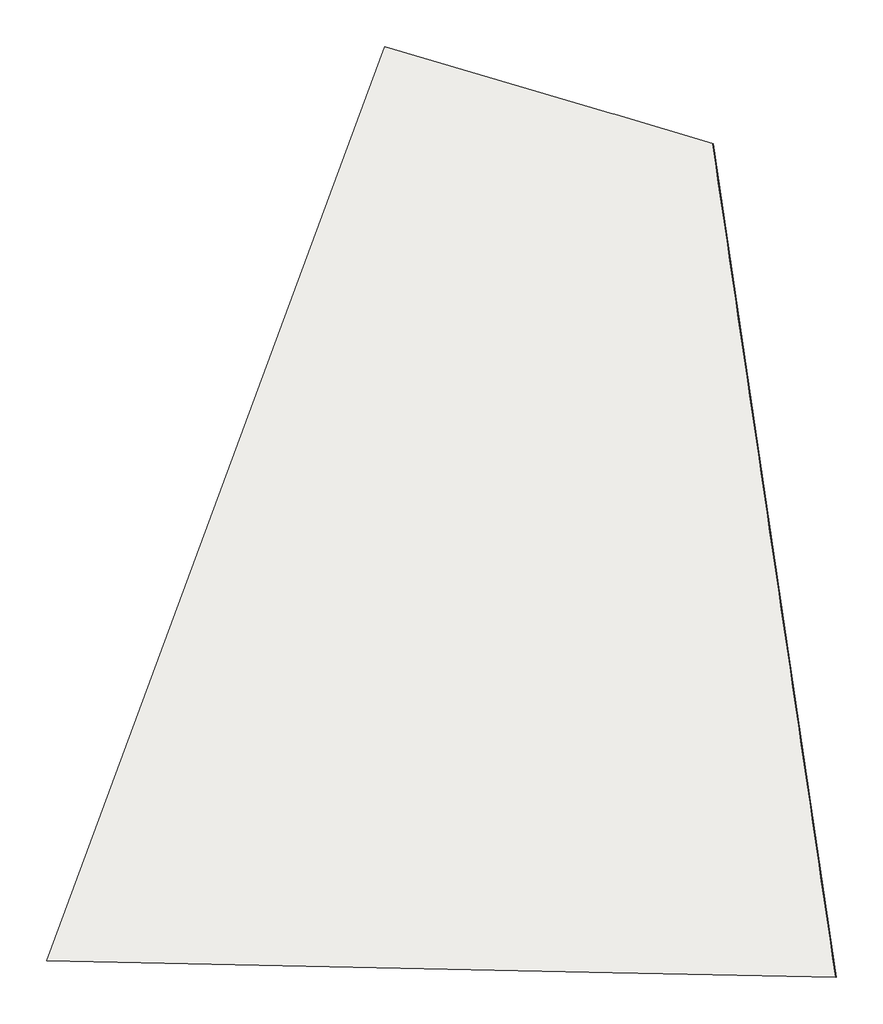
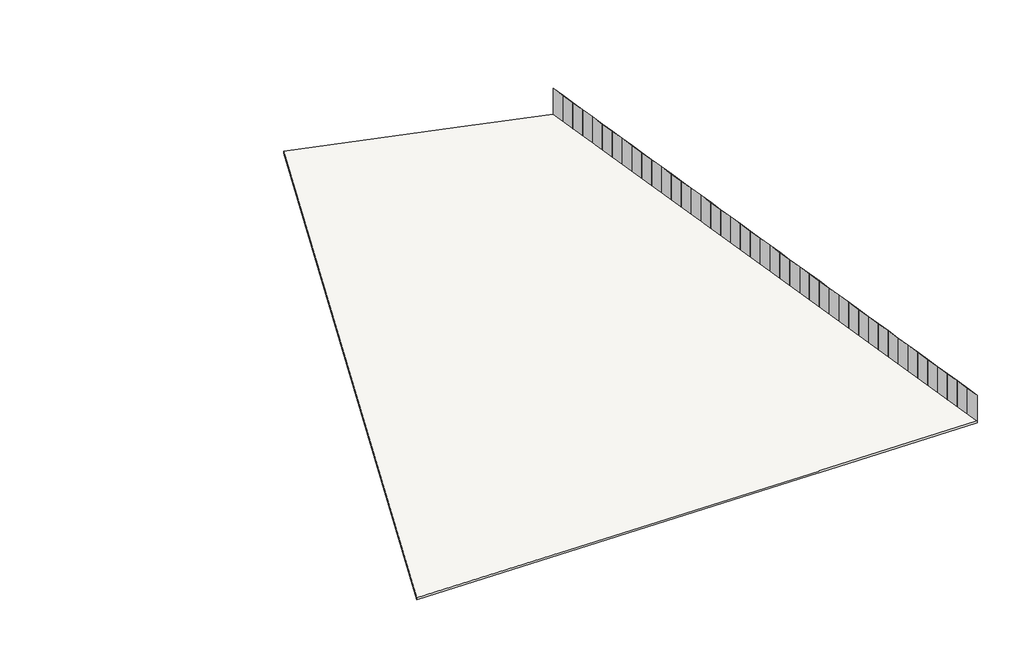
# One storey: 44 plates, 1 slab.
"""IFC4 building model written with IfcOpenShell, lengths in millimetres."""

import ifcopenshell
import ifcopenshell.guid

model = None  # the IFC model being written
_history = None  # IfcOwnerHistory: only IFC2X3 demands one
_inside = {}  # id of a spatial element -> (the spatial element, [elements in it])
_under = {}  # id of a project, library or spatial element -> (it, [spatial elements below it])
_declared = {}  # id of a project -> (the project, [libraries it declares])
_typed = {}  # id of a type object -> (the type object, [elements of that type])
_made_of = {}  # id of a material, layer set ... -> (it, [elements and type objects made of it])


def new_model(schema):
    """Start an empty IFC model of exactly this schema.

    Asked for "IFC4X3", IfcOpenShell would pick the latest addendum, in which some entities
    have other attributes; the version numbers below select the first issue.
    IFC2X3 requires an IfcOwnerHistory on every rooted entity: one is made here for all.
    """
    global model, _history
    if schema == "IFC4X3":
        model = ifcopenshell.file(schema_version=(4, 3, 0, 0))
    else:
        model = ifcopenshell.file(schema=schema)
    _inside.clear()
    _under.clear()
    _declared.clear()
    _typed.clear()
    _made_of.clear()
    _history = None
    if model.schema == "IFC2X3":
        org = make("IfcOrganization", Name="unknown")
        user = make(
            "IfcPersonAndOrganization",
            ThePerson=make("IfcPerson", FamilyName="unknown"),
            TheOrganization=org,
        )
        app = make(
            "IfcApplication",
            ApplicationDeveloper=org,
            Version="unknown",
            ApplicationFullName="unknown",
            ApplicationIdentifier="unknown",
        )
        _history = make(
            "IfcOwnerHistory",
            OwningUser=user,
            OwningApplication=app,
            ChangeAction="ADDED",
            CreationDate=0,
        )
    return model


def make(cls, **values):
    """One entity of the class cls with the attributes given. An attribute that is None is left unset."""
    return model.create_entity(
        cls, **{name: value for name, value in values.items() if value is not None}
    )


def rooted(cls, **values):
    """An entity with a GlobalId (a new one), such as an element, a storey or a relation."""
    return make(cls, GlobalId=ifcopenshell.guid.new(), OwnerHistory=_history, **values)


def si_unit(unit_type, name, prefix=None):
    """IfcSIUnit, for example si_unit("LENGTHUNIT", "METRE", prefix="MILLI")."""
    return make("IfcSIUnit", UnitType=unit_type, Prefix=prefix, Name=name)


def assignment(units):
    """IfcUnitAssignment: the units of a project."""
    return None if units is None else make("IfcUnitAssignment", Units=units)


def point(xyz):
    """IfcCartesianPoint."""
    return None if xyz is None else make("IfcCartesianPoint", Coordinates=xyz)


def direction(xyz):
    """IfcDirection."""
    return None if xyz is None else make("IfcDirection", DirectionRatios=xyz)


def frame(location, z_axis=None, x_axis=None):
    """IfcAxis2Placement3D, a coordinate frame: its origin and axes. An axis left out is left unset."""
    return make(
        "IfcAxis2Placement3D",
        Location=point(location),
        Axis=direction(z_axis),
        RefDirection=direction(x_axis),
    )


def origin():
    """The frame at (0, 0, 0) with its axes left unset."""
    return frame((0.0, 0.0, 0.0))


def origin_with_axes():
    """The frame at (0, 0, 0) with the z axis (0, 0, 1) and the x axis (1, 0, 0) written out."""
    return frame((0.0, 0.0, 0.0), z_axis=(0.0, 0.0, 1.0), x_axis=(1.0, 0.0, 0.0))


def place(relative_to, where):
    """IfcLocalPlacement: puts the frame where relative to a parent placement (None: the world)."""
    return make(
        "IfcLocalPlacement", PlacementRelTo=relative_to, RelativePlacement=where
    )


def context(
    kind, dimensions, precision=None, world=None, true_north=None, identifier=None
):
    """IfcGeometricRepresentationContext, for example the 3D "Model" context."""
    return make(
        "IfcGeometricRepresentationContext",
        ContextIdentifier=identifier,
        ContextType=kind,
        CoordinateSpaceDimension=dimensions,
        Precision=precision,
        WorldCoordinateSystem=world,
        TrueNorth=true_north,
    )


def project(units=None, contexts=None):
    """IfcProject with its units and contexts."""
    return rooted(
        "IfcProject",
        Name="project",
        RepresentationContexts=contexts,
        UnitsInContext=assignment(units),
    )


def spatial(cls, under=None, at=None, **own):
    """A site, building, storey or space (cls), placed at a placement, below another one or the project."""
    s = rooted(cls, ObjectPlacement=at, **own)
    if under is not None:
        _under.setdefault(under.id(), (under, []))[1].append(s)
    return s


def polyline(points):
    """IfcPolyline through the points."""
    return make("IfcPolyline", Points=[point(p) for p in points])


def outline(outer, holes=None, kind="AREA"):
    """IfcArbitraryClosedProfileDef: a profile drawn as a closed curve; with holes, ...WithVoids."""
    if holes is None:
        return make("IfcArbitraryClosedProfileDef", ProfileType=kind, OuterCurve=outer)
    return make(
        "IfcArbitraryProfileDefWithVoids",
        ProfileType=kind,
        OuterCurve=outer,
        InnerCurves=holes,
    )


def extrude(swept, where, along, depth):
    """IfcExtrudedAreaSolid: the profile swept, set in the frame where, extruded along a direction by depth."""
    return make(
        "IfcExtrudedAreaSolid",
        SweptArea=swept,
        Position=where,
        ExtrudedDirection=direction(along),
        Depth=depth,
    )


def faces_of(points, faces, orient=None, outer=None):
    """IfcFace entities. A face is a list of loops; a loop is a list of indices into points, from 0.

    orient and outer hold one flag for each loop. By default every Orientation is true, the
    first loop of a face is its IfcFaceOuterBound and the others are IfcFaceBound.
    """
    made = []
    for i, loops in enumerate(faces):
        bounds = []
        for j, loop in enumerate(loops):
            is_outer = j == 0 if outer is None else outer[i][j]
            bounds.append(
                make(
                    "IfcFaceOuterBound" if is_outer else "IfcFaceBound",
                    Bound=make("IfcPolyLoop", Polygon=[points[k] for k in loop]),
                    Orientation=True if orient is None else orient[i][j],
                )
            )
        made.append(make("IfcFace", Bounds=bounds))
    return made


def faceted_brep(points, faces, orient=None, outer=None, voids=None):
    """IfcFacetedBrep: a solid bounded by flat faces; with voids (closed shells), ...WithVoids."""
    shared = [point(p) for p in points]
    hull = make("IfcClosedShell", CfsFaces=faces_of(shared, faces, orient, outer))
    if voids is None:
        return make("IfcFacetedBrep", Outer=hull)
    return make(
        "IfcFacetedBrepWithVoids",
        Outer=hull,
        Voids=[
            make(cls, CfsFaces=faces_of(shared, fs, o, b)) for cls, fs, o, b in voids
        ],
    )


def shape(context_of_items, identifier, shape_type, items):
    """IfcShapeRepresentation: the items that make up one representation, for example the "Body"."""
    return make(
        "IfcShapeRepresentation",
        ContextOfItems=context_of_items,
        RepresentationIdentifier=identifier,
        RepresentationType=shape_type,
        Items=items,
    )


def source(mapping_origin, context_of_items, identifier, shape_type, items):
    """IfcRepresentationMap: a shape defined once, which mapped items show again and again."""
    return make(
        "IfcRepresentationMap",
        MappingOrigin=mapping_origin,
        MappedRepresentation=shape(context_of_items, identifier, shape_type, items),
    )


def transform(
    local_origin,
    x_axis=None,
    y_axis=None,
    z_axis=None,
    scale=None,
    scale2=None,
    scale3=None,
    uniform=True,
):
    """IfcCartesianTransformationOperator3D, or its non-uniform kind. x_axis, y_axis, z_axis: its Axis1, 2, 3."""
    if uniform:
        return make(
            "IfcCartesianTransformationOperator3D",
            Axis1=direction(x_axis),
            Axis2=direction(y_axis),
            LocalOrigin=point(local_origin),
            Scale=scale,
            Axis3=direction(z_axis),
        )
    return make(
        "IfcCartesianTransformationOperator3DnonUniform",
        Axis1=direction(x_axis),
        Axis2=direction(y_axis),
        LocalOrigin=point(local_origin),
        Scale=scale,
        Axis3=direction(z_axis),
        Scale2=scale2,
        Scale3=scale3,
    )


def mapped(mapping_source, mapping_target):
    """IfcMappedItem: shows the shape of a source again, moved by a transform."""
    return make(
        "IfcMappedItem", MappingSource=mapping_source, MappingTarget=mapping_target
    )


def made_of(thing, what):
    """Note that an element or type object is made of a material, layer set ...; save() writes the relation."""
    if what is not None:
        _made_of.setdefault(what.id(), (what, []))[1].append(thing)
    return thing


def element(
    cls,
    number,
    at=None,
    inside=None,
    cuts=None,
    type_object=None,
    material=None,
    context=None,
    identifier="Body",
    shape_type=None,
    held_by="IfcProductDefinitionShape",
    body=None,
    shapes=None,
    **own,
):
    """One element of the class cls, such as IfcWall. Its Tag is "e" and its number.

    at: its placement. inside: the storey or other place that contains it. cuts: it is an
    opening in that element (IfcRelVoidsElement). A single representation is given by context,
    identifier, shape_type and body (its items); several are given by shapes. held_by: the class
    of the entity that holds the representations. save() writes the other relations.
    """
    e = rooted(cls, Tag="e%d" % number, ObjectPlacement=at, **own)
    if body is not None:
        shapes = [shape(context, identifier, shape_type, body)]
    if shapes is not None:
        e.Representation = make(held_by, Representations=shapes)
    if inside is not None:
        _inside.setdefault(inside.id(), (inside, []))[1].append(e)
    if cuts is not None:
        rooted(
            "IfcRelVoidsElement", RelatingBuildingElement=cuts, RelatedOpeningElement=e
        )
    if type_object is not None:
        _typed.setdefault(type_object.id(), (type_object, []))[1].append(e)
    return made_of(e, material)


def aggregate(whole, parts):
    """IfcRelAggregates: a whole, such as a stair, and the parts it consists of."""
    return rooted("IfcRelAggregates", RelatingObject=whole, RelatedObjects=parts)


def save(model, path):
    """Write the relations noted so far, then the file.

    IfcRelAggregates (storeys below a building ...), IfcRelContainedInSpatialStructure (elements
    in a storey), IfcRelDefinesByType, IfcRelAssociatesMaterial and IfcRelDeclares: one each for
    every whole, place, type object, material and project.
    """
    for whole, parts in _under.values():
        aggregate(whole, parts)
    for where, things in _inside.values():
        rooted(
            "IfcRelContainedInSpatialStructure",
            RelatedElements=things,
            RelatingStructure=where,
        )
    for kind, things in _typed.values():
        rooted("IfcRelDefinesByType", RelatedObjects=things, RelatingType=kind)
    for what, things in _made_of.values():
        rooted("IfcRelAssociatesMaterial", RelatedObjects=things, RelatingMaterial=what)
    for by, libraries in _declared.values():
        rooted("IfcRelDeclares", RelatingContext=by, RelatedDefinitions=libraries)
    model.write(path)


def painel_do_sistema_1cdad03e(model_context):
    return source(origin(), model_context, "Body", "SweptSolid", [
        extrude(outline(polyline([(1500.0, 24.5), (-1500.0, 24.5), (-1500.0, 49.5), (1500.0, 49.5), (1500.0, 24.5)])), origin_with_axes(), (0.0, 0.0, 1.0), 1500.0),
    ])


def painel_do_sistema_1cb3a730(model_context):
    return source(origin(), model_context, "Body", "SweptSolid", [
        extrude(outline(polyline([(1500.0, 24.5), (-1500.0, 24.5), (-1500.0, 49.5), (1500.0, 49.5), (1500.0, 24.5)])), origin_with_axes(), (0.0, 0.0, 1.0), 20.0931032),
    ])


model = new_model("IFC4")

# Units and contexts
model_context = context("Model", 3, world=origin())
ifc_project = project(units=[si_unit("LENGTHUNIT", "METRE", prefix="MILLI")], contexts=[model_context])

# Site, building, storey
site = spatial("IfcSite", under=ifc_project)
building = spatial("IfcBuilding", under=site)
storey = spatial("IfcBuildingStorey", under=building, Name="Nível 7", Elevation=6000.0)

# Plates
placement = place(None, origin())
painel_do_sistema_shape = painel_do_sistema_1cdad03e(model_context)
element("IfcPlate", 1, ObjectType="Painel do sistema : Envidraçado", at=placement, inside=storey, context=model_context, shape_type="MappedRepresentation", body=[
    mapped(painel_do_sistema_shape, transform((27835.0106579, -36774.1442579, 7500.000015), x_axis=(0.0, 0.0, 1.0), y_axis=(-0.9892699032546327, -0.1460994815684493, 0.0), z_axis=(0.1460994815684493, -0.9892699032546327, 0.0))),
])
element("IfcPlate", 2, ObjectType="Painel do sistema : Envidraçado", at=placement, inside=storey, context=model_context, shape_type="MappedRepresentation", body=[
    mapped(painel_do_sistema_shape, transform((27615.8614356, -35290.239403, 7500.000015), x_axis=(0.0, 0.0, 1.0), y_axis=(-0.9892699032546328, -0.14609948156844885, 0.0), z_axis=(0.14609948156844885, -0.9892699032546328, 0.0))),
])
element("IfcPlate", 3, ObjectType="Painel do sistema : Envidraçado", at=placement, inside=storey, context=model_context, shape_type="MappedRepresentation", body=[
    mapped(painel_do_sistema_shape, transform((27396.7122132, -33806.3345481, 7500.000015), x_axis=(0.0, 0.0, 1.0), y_axis=(-0.9892699032546323, -0.1460994815684521, 0.0), z_axis=(0.1460994815684521, -0.9892699032546323, 0.0))),
])
element("IfcPlate", 4, ObjectType="Painel do sistema : Envidraçado", at=placement, inside=storey, context=model_context, shape_type="MappedRepresentation", body=[
    mapped(painel_do_sistema_shape, transform((27177.5629909, -32322.4296932, 7500.000015), x_axis=(0.0, 0.0, 1.0), y_axis=(-0.9892699032546328, -0.14609948156844926, 0.0), z_axis=(0.14609948156844926, -0.9892699032546328, 0.0))),
])
element("IfcPlate", 5, ObjectType="Painel do sistema : Envidraçado", at=placement, inside=storey, context=model_context, shape_type="MappedRepresentation", body=[
    mapped(painel_do_sistema_shape, transform((26958.4137685, -30838.5248383, 7500.000015), x_axis=(0.0, 0.0, 1.0), y_axis=(-0.9892699032546327, -0.1460994815684493, 0.0), z_axis=(0.1460994815684493, -0.9892699032546327, 0.0))),
])
element("IfcPlate", 6, ObjectType="Painel do sistema : Envidraçado", at=placement, inside=storey, context=model_context, shape_type="MappedRepresentation", body=[
    mapped(painel_do_sistema_shape, transform((26739.2645462, -29354.6199835, 7500.000015), x_axis=(0.0, 0.0, 1.0), y_axis=(-0.9892699032546327, -0.1460994815684493, 0.0), z_axis=(0.1460994815684493, -0.9892699032546327, 0.0))),
])
element("IfcPlate", 7, ObjectType="Painel do sistema : Envidraçado", at=placement, inside=storey, context=model_context, shape_type="MappedRepresentation", body=[
    mapped(painel_do_sistema_shape, transform((26520.1153238, -27870.7151286, 7500.000015), x_axis=(0.0, 0.0, 1.0), y_axis=(-0.9892699032546324, -0.1460994815684517, 0.0), z_axis=(0.1460994815684517, -0.9892699032546324, 0.0))),
])
element("IfcPlate", 8, ObjectType="Painel do sistema : Envidraçado", at=placement, inside=storey, context=model_context, shape_type="MappedRepresentation", body=[
    mapped(painel_do_sistema_shape, transform((26300.9661014, -26386.8102737, 7500.000015), x_axis=(0.0, 0.0, 1.0), y_axis=(-0.9892699032546327, -0.1460994815684493, 0.0), z_axis=(0.1460994815684493, -0.9892699032546327, 0.0))),
])
element("IfcPlate", 9, ObjectType="Painel do sistema : Envidraçado", at=placement, inside=storey, context=model_context, shape_type="MappedRepresentation", body=[
    mapped(painel_do_sistema_shape, transform((26081.8168791, -24902.9054188, 7500.000015), x_axis=(0.0, 0.0, 1.0), y_axis=(-0.9892699032546328, -0.14609948156844887, 0.0), z_axis=(0.14609948156844887, -0.9892699032546328, 0.0))),
])
element("IfcPlate", 10, ObjectType="Painel do sistema : Envidraçado", at=placement, inside=storey, context=model_context, shape_type="MappedRepresentation", body=[
    mapped(painel_do_sistema_shape, transform((25862.6676567, -23419.0005639, 7500.000015), x_axis=(0.0, 0.0, 1.0), y_axis=(-0.9892699032546324, -0.1460994815684517, 0.0), z_axis=(0.1460994815684517, -0.9892699032546324, 0.0))),
])
element("IfcPlate", 11, ObjectType="Painel do sistema : Envidraçado", at=placement, inside=storey, context=model_context, shape_type="MappedRepresentation", body=[
    mapped(painel_do_sistema_shape, transform((25643.5184344, -21935.095709, 7500.000015), x_axis=(0.0, 0.0, 1.0), y_axis=(-0.9892699032546327, -0.14609948156844926, 0.0), z_axis=(0.14609948156844926, -0.9892699032546327, 0.0))),
])
element("IfcPlate", 12, ObjectType="Painel do sistema : Envidraçado", at=placement, inside=storey, context=model_context, shape_type="MappedRepresentation", body=[
    mapped(painel_do_sistema_shape, transform((25424.369212, -20451.1908542, 7500.000015), x_axis=(0.0, 0.0, 1.0), y_axis=(-0.9892699032546324, -0.1460994815684517, 0.0), z_axis=(0.1460994815684517, -0.9892699032546324, 0.0))),
])
element("IfcPlate", 13, ObjectType="Painel do sistema : Envidraçado", at=placement, inside=storey, context=model_context, shape_type="MappedRepresentation", body=[
    mapped(painel_do_sistema_shape, transform((25205.2199897, -18967.2859993, 7500.000015), x_axis=(0.0, 0.0, 1.0), y_axis=(-0.9892699032546328, -0.14609948156844865, 0.0), z_axis=(0.14609948156844865, -0.9892699032546328, 0.0))),
])
element("IfcPlate", 14, ObjectType="Painel do sistema : Envidraçado", at=placement, inside=storey, context=model_context, shape_type="MappedRepresentation", body=[
    mapped(painel_do_sistema_shape, transform((24986.0707673, -17483.3811444, 7500.000015), x_axis=(0.0, 0.0, 1.0), y_axis=(-0.9892699032546328, -0.1460994815684491, 0.0), z_axis=(0.1460994815684491, -0.9892699032546328, 0.0))),
])
element("IfcPlate", 15, ObjectType="Painel do sistema : Envidraçado", at=placement, inside=storey, context=model_context, shape_type="MappedRepresentation", body=[
    mapped(painel_do_sistema_shape, transform((24766.921545, -15999.4762895, 7500.000015), x_axis=(0.0, 0.0, 1.0), y_axis=(-0.9892699032546327, -0.1460994815684493, 0.0), z_axis=(0.1460994815684493, -0.9892699032546327, 0.0))),
])
element("IfcPlate", 16, ObjectType="Painel do sistema : Envidraçado", at=placement, inside=storey, context=model_context, shape_type="MappedRepresentation", body=[
    mapped(painel_do_sistema_shape, transform((24547.7723226, -14515.5714346, 7500.000015), x_axis=(0.0, 0.0, 1.0), y_axis=(-0.9892699032546324, -0.1460994815684517, 0.0), z_axis=(0.1460994815684517, -0.9892699032546324, 0.0))),
])
element("IfcPlate", 17, ObjectType="Painel do sistema : Envidraçado", at=placement, inside=storey, context=model_context, shape_type="MappedRepresentation", body=[
    mapped(painel_do_sistema_shape, transform((24328.6231003, -13031.6665798, 7500.000015), x_axis=(0.0, 0.0, 1.0), y_axis=(-0.9892699032546327, -0.1460994815684495, 0.0), z_axis=(0.1460994815684495, -0.9892699032546327, 0.0))),
])
element("IfcPlate", 18, ObjectType="Painel do sistema : Envidraçado", at=placement, inside=storey, context=model_context, shape_type="MappedRepresentation", body=[
    mapped(painel_do_sistema_shape, transform((24109.4738779, -11547.7617249, 7500.000015), x_axis=(0.0, 0.0, 1.0), y_axis=(-0.9892699032546328, -0.1460994815684491, 0.0), z_axis=(0.1460994815684491, -0.9892699032546328, 0.0))),
])
element("IfcPlate", 19, ObjectType="Painel do sistema : Envidraçado", at=placement, inside=storey, context=model_context, shape_type="MappedRepresentation", body=[
    mapped(painel_do_sistema_shape, transform((23890.3246556, -10063.85687, 7500.000015), x_axis=(0.0, 0.0, 1.0), y_axis=(-0.9892699032546324, -0.14609948156845148, 0.0), z_axis=(0.14609948156845148, -0.9892699032546324, 0.0))),
])
element("IfcPlate", 20, ObjectType="Painel do sistema : Envidraçado", at=placement, inside=storey, context=model_context, shape_type="MappedRepresentation", body=[
    mapped(painel_do_sistema_shape, transform((23671.1754332, -8579.9520151, 7500.000015), x_axis=(0.0, 0.0, 1.0), y_axis=(-0.9892699032546332, -0.14609948156844624, 0.0), z_axis=(0.14609948156844624, -0.9892699032546332, 0.0))),
])
element("IfcPlate", 21, ObjectType="Painel do sistema : Envidraçado", at=placement, inside=storey, context=model_context, shape_type="MappedRepresentation", body=[
    mapped(painel_do_sistema_shape, transform((23452.0262109, -7096.0471602, 7500.000015), x_axis=(0.0, 0.0, 1.0), y_axis=(-0.9892699032546319, -0.14609948156845473, 0.0), z_axis=(0.14609948156845473, -0.9892699032546319, 0.0))),
])
element("IfcPlate", 22, ObjectType="Painel do sistema : Envidraçado", at=placement, inside=storey, context=model_context, shape_type="MappedRepresentation", body=[
    mapped(painel_do_sistema_shape, transform((23232.8769885, -5612.1423053, 7500.000015), x_axis=(0.0, 0.0, 1.0), y_axis=(-0.9892699032546332, -0.1460994815684465, 0.0), z_axis=(0.1460994815684465, -0.9892699032546332, 0.0))),
])
element("IfcPlate", 23, ObjectType="Painel do sistema : Envidraçado", at=placement, inside=storey, context=model_context, shape_type="MappedRepresentation", body=[
    mapped(painel_do_sistema_shape, transform((23013.7277662, -4128.2374505, 7500.000015), x_axis=(0.0, 0.0, 1.0), y_axis=(-0.9892699032546324, -0.1460994815684517, 0.0), z_axis=(0.1460994815684517, -0.9892699032546324, 0.0))),
])
element("IfcPlate", 24, ObjectType="Painel do sistema : Envidraçado", at=placement, inside=storey, context=model_context, shape_type="MappedRepresentation", body=[
    mapped(painel_do_sistema_shape, transform((22794.5785438, -2644.3325956, 7500.000015), x_axis=(0.0, 0.0, 1.0), y_axis=(-0.9892699032546328, -0.14609948156844865, 0.0), z_axis=(0.14609948156844865, -0.9892699032546328, 0.0))),
])
element("IfcPlate", 25, ObjectType="Painel do sistema : Envidraçado", at=placement, inside=storey, context=model_context, shape_type="MappedRepresentation", body=[
    mapped(painel_do_sistema_shape, transform((22575.4293215, -1160.4277407, 7500.000015), x_axis=(0.0, 0.0, 1.0), y_axis=(-0.9892699032546327, -0.1460994815684493, 0.0), z_axis=(0.1460994815684493, -0.9892699032546327, 0.0))),
])
element("IfcPlate", 26, ObjectType="Painel do sistema : Envidraçado", at=placement, inside=storey, context=model_context, shape_type="MappedRepresentation", body=[
    mapped(painel_do_sistema_shape, transform((22356.2800991, 323.4771142, 7500.000015), x_axis=(0.0, 0.0, 1.0), y_axis=(-0.9892699032546324, -0.14609948156845148, 0.0), z_axis=(0.14609948156845148, -0.9892699032546324, 0.0))),
])
element("IfcPlate", 27, ObjectType="Painel do sistema : Envidraçado", at=placement, inside=storey, context=model_context, shape_type="MappedRepresentation", body=[
    mapped(painel_do_sistema_shape, transform((22137.1308767, 1807.3819691, 7500.000015), x_axis=(0.0, 0.0, 1.0), y_axis=(-0.9892699032546332, -0.1460994815684469, 0.0), z_axis=(0.1460994815684469, -0.9892699032546332, 0.0))),
])
element("IfcPlate", 28, ObjectType="Painel do sistema : Envidraçado", at=placement, inside=storey, context=model_context, shape_type="MappedRepresentation", body=[
    mapped(painel_do_sistema_shape, transform((21917.9816544, 3291.2868239, 7500.000015), x_axis=(0.0, 0.0, 1.0), y_axis=(-0.9892699032546323, -0.1460994815684521, 0.0), z_axis=(0.1460994815684521, -0.9892699032546323, 0.0))),
])
element("IfcPlate", 29, ObjectType="Painel do sistema : Envidraçado", at=placement, inside=storey, context=model_context, shape_type="MappedRepresentation", body=[
    mapped(painel_do_sistema_shape, transform((21698.832432, 4775.1916788, 7500.000015), x_axis=(0.0, 0.0, 1.0), y_axis=(-0.9892699032546323, -0.14609948156845234, 0.0), z_axis=(0.14609948156845234, -0.9892699032546323, 0.0))),
])
element("IfcPlate", 30, ObjectType="Painel do sistema : Envidraçado", at=placement, inside=storey, context=model_context, shape_type="MappedRepresentation", body=[
    mapped(painel_do_sistema_shape, transform((21479.6832097, 6259.0965337, 7500.000015), x_axis=(0.0, 0.0, 1.0), y_axis=(-0.9892699032546332, -0.1460994815684465, 0.0), z_axis=(0.1460994815684465, -0.9892699032546332, 0.0))),
])
element("IfcPlate", 31, ObjectType="Painel do sistema : Envidraçado", at=placement, inside=storey, context=model_context, shape_type="MappedRepresentation", body=[
    mapped(painel_do_sistema_shape, transform((21260.5339873, 7743.0013886, 7500.000015), x_axis=(0.0, 0.0, 1.0), y_axis=(-0.9892699032546323, -0.14609948156845234, 0.0), z_axis=(0.14609948156845234, -0.9892699032546323, 0.0))),
])
element("IfcPlate", 32, ObjectType="Painel do sistema : Envidraçado", at=placement, inside=storey, context=model_context, shape_type="MappedRepresentation", body=[
    mapped(painel_do_sistema_shape, transform((21041.384765, 9226.9062435, 7500.000015), x_axis=(0.0, 0.0, 1.0), y_axis=(-0.9892699032546327, -0.1460994815684495, 0.0), z_axis=(0.1460994815684495, -0.9892699032546327, 0.0))),
])
element("IfcPlate", 33, ObjectType="Painel do sistema : Envidraçado", at=placement, inside=storey, context=model_context, shape_type="MappedRepresentation", body=[
    mapped(painel_do_sistema_shape, transform((20822.2355426, 10710.8110984, 7500.000015), x_axis=(0.0, 0.0, 1.0), y_axis=(-0.9892699032546327, -0.1460994815684495, 0.0), z_axis=(0.1460994815684495, -0.9892699032546327, 0.0))),
])
element("IfcPlate", 34, ObjectType="Painel do sistema : Envidraçado", at=placement, inside=storey, context=model_context, shape_type="MappedRepresentation", body=[
    mapped(painel_do_sistema_shape, transform((20603.0863203, 12194.7159532, 7500.000015), x_axis=(0.0, 0.0, 1.0), y_axis=(-0.9892699032546327, -0.1460994815684495, 0.0), z_axis=(0.1460994815684495, -0.9892699032546327, 0.0))),
])
element("IfcPlate", 35, ObjectType="Painel do sistema : Envidraçado", at=placement, inside=storey, context=model_context, shape_type="MappedRepresentation", body=[
    mapped(painel_do_sistema_shape, transform((20383.9370979, 13678.6208081, 7500.000015), x_axis=(0.0, 0.0, 1.0), y_axis=(-0.9892699032546326, -0.14609948156845054, 0.0), z_axis=(0.14609948156845054, -0.9892699032546326, 0.0))),
])
element("IfcPlate", 36, ObjectType="Painel do sistema : Envidraçado", at=placement, inside=storey, context=model_context, shape_type="MappedRepresentation", body=[
    mapped(painel_do_sistema_shape, transform((20164.7878756, 15162.525663, 7500.000015), x_axis=(0.0, 0.0, 1.0), y_axis=(-0.9892699032546328, -0.14609948156844887, 0.0), z_axis=(0.14609948156844887, -0.9892699032546328, 0.0))),
])
element("IfcPlate", 37, ObjectType="Painel do sistema : Envidraçado", at=placement, inside=storey, context=model_context, shape_type="MappedRepresentation", body=[
    mapped(painel_do_sistema_shape, transform((19945.6386532, 16646.4305179, 7500.000015), x_axis=(0.0, 0.0, 1.0), y_axis=(-0.9892699032546327, -0.1460994815684493, 0.0), z_axis=(0.1460994815684493, -0.9892699032546327, 0.0))),
])
element("IfcPlate", 38, ObjectType="Painel do sistema : Envidraçado", at=placement, inside=storey, context=model_context, shape_type="MappedRepresentation", body=[
    mapped(painel_do_sistema_shape, transform((19726.4894309, 18130.3353728, 7500.000015), x_axis=(0.0, 0.0, 1.0), y_axis=(-0.9892699032546326, -0.14609948156845012, 0.0), z_axis=(0.14609948156845012, -0.9892699032546326, 0.0))),
])
element("IfcPlate", 39, ObjectType="Painel do sistema : Envidraçado", at=placement, inside=storey, context=model_context, shape_type="MappedRepresentation", body=[
    mapped(painel_do_sistema_shape, transform((19507.3402085, 19614.2402276, 7500.000015), x_axis=(0.0, 0.0, 1.0), y_axis=(-0.9892699032546329, -0.14609948156844849, 0.0), z_axis=(0.14609948156844849, -0.9892699032546329, 0.0))),
])
element("IfcPlate", 40, ObjectType="Painel do sistema : Envidraçado", at=placement, inside=storey, context=model_context, shape_type="MappedRepresentation", body=[
    mapped(painel_do_sistema_shape, transform((19288.1909862, 21098.1450825, 7500.000015), x_axis=(0.0, 0.0, 1.0), y_axis=(-0.9892699032546323, -0.14609948156845254, 0.0), z_axis=(0.14609948156845254, -0.9892699032546323, 0.0))),
])
element("IfcPlate", 41, ObjectType="Painel do sistema : Envidraçado", at=placement, inside=storey, context=model_context, shape_type="MappedRepresentation", body=[
    mapped(painel_do_sistema_shape, transform((19069.0417638, 22582.0499374, 7500.000015), x_axis=(0.0, 0.0, 1.0), y_axis=(-0.9892699032546326, -0.1460994815684497, 0.0), z_axis=(0.1460994815684497, -0.9892699032546326, 0.0))),
])
element("IfcPlate", 42, ObjectType="Painel do sistema : Envidraçado", at=placement, inside=storey, context=model_context, shape_type="MappedRepresentation", body=[
    mapped(painel_do_sistema_shape, transform((18849.8925415, 24065.9547923, 7500.000015), x_axis=(0.0, 0.0, 1.0), y_axis=(-0.9892699032546326, -0.14609948156845012, 0.0), z_axis=(0.14609948156845012, -0.9892699032546326, 0.0))),
])
element("IfcPlate", 43, ObjectType="Painel do sistema : Envidraçado", at=placement, inside=storey, context=model_context, shape_type="MappedRepresentation", body=[
    mapped(painel_do_sistema_shape, transform((18630.7433191, 25549.8596472, 7500.000015), x_axis=(0.0, 0.0, 1.0), y_axis=(-0.9892699032546327, -0.14609948156844987, 0.0), z_axis=(0.14609948156844987, -0.9892699032546327, 0.0))),
])
painel_do_sistema_2_shape = painel_do_sistema_1cb3a730(model_context)
element("IfcPlate", 44, ObjectType="Painel do sistema : Envidraçado", at=placement, inside=storey, context=model_context, shape_type="MappedRepresentation", body=[
    mapped(painel_do_sistema_2_shape, transform((18627.8077271, 25569.7371494, 7500.000015), x_axis=(0.0, 0.0, 1.0), y_axis=(-0.9892699032546369, -0.14609948156842115, 0.0), z_axis=(0.14609948156842115, -0.9892699032546369, 0.0))),
])

# Slab
element("IfcSlab", 45, ObjectType="piso aula 04", at=placement, inside=storey, context=model_context, shape_type="Brep", body=[
    faceted_brep([(18627.8077271, 25569.7371494, 5790.0), (28054.1598803, -38258.0491127, 5790.0), (10995.3657537, -37899.7374539, 5790.0), (10920.3657537, -37898.1621155, 5790.0), (-32413.6745309, -36987.9517137, 5790.0), (-6526.0277886, 32996.9225357, 5790.0), (10995.3657537, 27823.3720454, 5790.0), (11070.3657537, 27801.2267585, 5790.0), (18627.8077271, 25569.7371494, 6000.0), (11070.3657537, 27801.2267585, 6000.0), (10995.3657537, 27823.3720454, 6000.0), (-6526.0277886, 32996.9225357, 6000.0), (-32413.6745309, -36987.9517137, 6000.0), (10920.3657537, -37898.1621155, 6000.0), (10995.3657537, -37899.7374539, 6000.0), (28054.1598803, -38258.0491127, 6000.0)], [[[0, 1, 2, 3, 4, 5, 6, 7]], [[8, 9, 10, 11, 12, 13, 14, 15]], [[1, 0, 8, 15]], [[4, 3, 2, 1, 15, 14, 13, 12]], [[5, 4, 12, 11]], [[0, 7, 6, 5, 11, 10, 9, 8]]]),
])

save(model, "model.ifc")

# Revit data of these elements
# Type "Painel do sistema : Envidraçado"
#   Construction Type Id = "GSP4R"
#   Analytic Construction = "Vidraça única Pilkington 1/8 pol"
#   Visual Light Transmittance = 0.9
#   Solar Heat Gain Coefficient = 0.86
#   Heat Transfer Coefficient (U) = 6.7069 W/(m²·K)
# Type "piso aula 04"
#   Function = 0
#   Layers, outside or top first: 0.02 m "Azulejo cerâmico" (function 4); 0.04 m "Concreto, Faixa de areia/cimento" (function 2); 0.15 m "Concreto,  Moldado in loco" (function 1)
# Elements 1, 2, 3, 4, 5, 6, 7, 8, 9, 10, 11, 12, 13, 14, 15, 16, 17, 18, 19, 20, 21, 22, 23, 24, 25, 26, 27, 28, 29, 30, 31, 32, 33, 34, 35, 36, 37, 38, 39, 40, 41, 42, 43, 44 (IfcPlate, "Painel do sistema : Envidraçado")
#   Phase Created = Construção nova
#   Materials on its faces: "Vidro"
# Element 45 (IfcSlab, "piso aula 04")
#   built-in parameter 1001955 = -0.287112 (stored number, unit not read)
#   Height Offset From Level = 0.00 m
#   Phase Created = Construção nova
#   Materials on its faces: "Concreto,  Moldado in loco", "Azulejo cerâmico"
# Materials
#   "Azulejo cerâmico": class "Cerâmica", colour RGB 246 230 196, transparency 0, Description = "Material físico", Cost = 0
#   "Concreto, Faixa de areia/cimento": class "Concreto", colour RGB 127 127 127, transparency 0, Description = "Revestimento de laje de concreto", Cost = 0
#   "Concreto,  Moldado in loco": class "Concreto", colour RGB 192 192 192, transparency 0, Description = "Material físico", Cost = 0
#   "Vidro": class "Vidro", colour RGB 0 128 192, transparency 0.9, Description = "Vidro de sílica", Cost = 0
